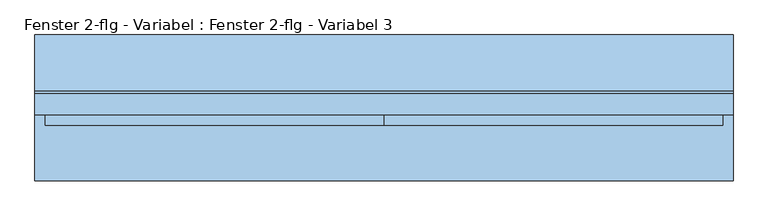
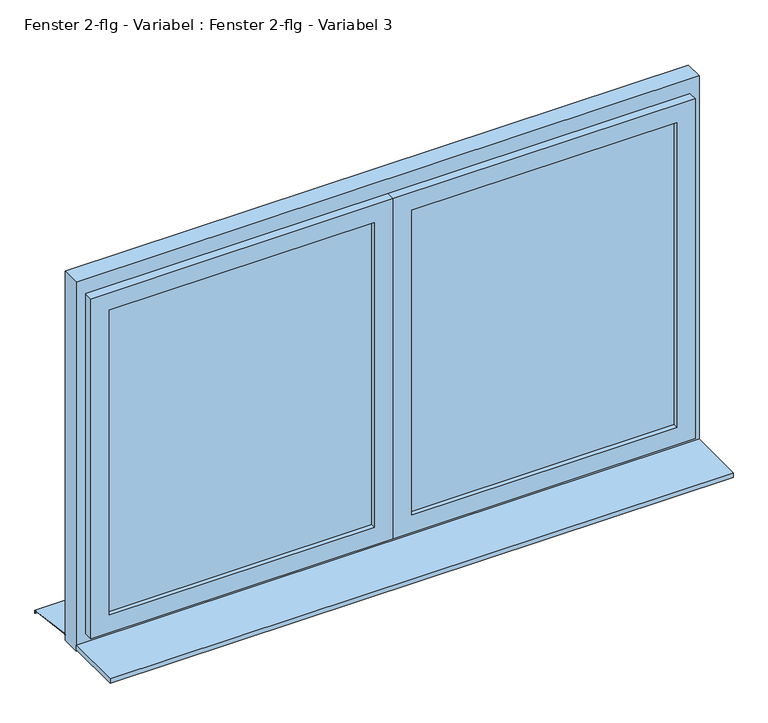
"""IFC4 building model written with IfcOpenShell, lengths in millimetres: window geometry, Fenster 2-flg - Variabel : Fenster 2-flg - Variabel 3."""

from ifc_helpers import new_model, si_unit, frame, origin, place, context, project, spatial, polyline, outline, extrude, faceted_brep, source, transform, mapped, element, save


def fenster_2_flg_variabel_fenster_2_flg_variabel_3_03287464(model_context):
    return source(origin(), model_context, "Body", "SolidModel", [
        extrude(outline(polyline([(60.0, -5.0), (915.0, -5.0), (915.0, -35.0), (60.0, -35.0), (60.0, -5.0)])), frame((0.0, 0.0, 1110.0), z_axis=(0.0, 0.0, 1.0), x_axis=(1.0, 0.0, 0.0)), (0.0, 0.0, 1.0), 1040.0),
        extrude(outline(polyline([(-915.0, -5.0), (-60.0, -5.0), (-60.0, -35.0), (-915.0, -35.0), (-915.0, -5.0)])), frame((0.0, 0.0, 1110.0), z_axis=(0.0, 0.0, 1.0), x_axis=(1.0, 0.0, 0.0)), (0.0, 0.0, 1.0), 1040.0),
        extrude(outline(polyline([(-1005.0, -210.0), (-1005.0, -20.0), (1005.0, -20.0), (1005.0, -210.0), (-1005.0, -210.0)])), frame((0.0, 0.0, 1005.0), z_axis=(0.0, 0.0, 1.0), x_axis=(1.0, 0.0, 0.0)), (0.0, 0.0, 1.0), 15.0),
        extrude(outline(polyline([(50.0221543, 1020.0), (210.0, 1000.0), (210.0, 990.0), (208.0, 990.0), (208.0, 998.3604634), (49.8240723, 1018.0), (40.0, 1018.0), (40.0, 1020.0), (50.0221543, 1020.0)])), frame((-1005.0, 0.0, 0.0), z_axis=(1.0, 0.0, 0.0), x_axis=(0.0, 1.0, 0.0)), (0.0, 0.0, 1.0), 2010.0),
        extrude(outline(polyline([(30.0, -20.0), (-30.0, -20.0), (-30.0, 40.0), (30.0, 40.0), (30.0, -20.0)])), frame((0.0, 0.0, 1080.0), z_axis=(0.0, 0.0, 1.0), x_axis=(1.0, 0.0, 0.0)), (0.0, 0.0, 1.0), 1100.0),
        extrude(outline(polyline([(2260.0, -1005.0), (1000.0, -1005.0), (1000.0, 1005.0), (2260.0, 1005.0), (2260.0, -1005.0)]), holes=[polyline([(2180.0, -945.0), (2180.0, 945.0), (1080.0, 945.0), (1080.0, -945.0), (2180.0, -945.0)])]), frame((0.0, -20.0, 0.0), z_axis=(0.0, 1.0, 0.0), x_axis=(0.0, 0.0, 1.0)), (0.0, 0.0, 1.0), 60.0),
        faceted_brep([(-945.0, -20.0, 1080.0), (-945.0, 10.0, 1080.0), (-30.0, 10.0, 1080.0), (-30.0, -20.0, 1080.0), (-30.0, 10.0, 2180.0), (-30.0, -20.0, 2180.0), (-945.0, 10.0, 2180.0), (-60.0, 10.0, 2150.0), (-915.0, 10.0, 2150.0), (-915.0, 10.0, 1110.0), (-60.0, 10.0, 1110.0), (0.0, -20.0, 1050.0), (-975.0, -20.0, 1050.0), (-975.0, -20.0, 2210.0), (0.0, -20.0, 2210.0), (-945.0, -20.0, 2180.0), (-975.0, -50.0, 1050.0), (0.0, -50.0, 1050.0), (0.0, -50.0, 2210.0), (-975.0, -50.0, 2210.0), (-60.0, -50.0, 1110.0), (-915.0, -50.0, 1110.0), (-915.0, -50.0, 2150.0), (-60.0, -50.0, 2150.0)], [[[0, 1, 2, 3]], [[3, 2, 4, 5]], [[2, 1, 6, 4], [7, 8, 9, 10]], [[11, 12, 13, 14], [5, 15, 0, 3]], [[16, 12, 11, 17]], [[17, 11, 14, 18]], [[18, 19, 16, 17], [20, 21, 22, 23]], [[9, 21, 20, 10]], [[10, 20, 23, 7]], [[15, 6, 1, 0]], [[19, 13, 12, 16]], [[8, 22, 21, 9]], [[5, 4, 6, 15]], [[18, 14, 13, 19]], [[7, 23, 22, 8]]]),
        faceted_brep([(30.0, -20.0, 1080.0), (30.0, 10.0, 1080.0), (945.0, 10.0, 1080.0), (945.0, -20.0, 1080.0), (945.0, 10.0, 2180.0), (945.0, -20.0, 2180.0), (30.0, 10.0, 2180.0), (915.0, 10.0, 2150.0), (60.0, 10.0, 2150.0), (60.0, 10.0, 1110.0), (915.0, 10.0, 1110.0), (975.0, -20.0, 1050.0), (0.0, -20.0, 1050.0), (0.0, -20.0, 2210.0), (975.0, -20.0, 2210.0), (30.0, -20.0, 2180.0), (0.0, -50.0, 1050.0), (975.0, -50.0, 1050.0), (975.0, -50.0, 2210.0), (0.0, -50.0, 2210.0), (915.0, -50.0, 1110.0), (60.0, -50.0, 1110.0), (60.0, -50.0, 2150.0), (915.0, -50.0, 2150.0)], [[[0, 1, 2, 3]], [[3, 2, 4, 5]], [[2, 1, 6, 4], [7, 8, 9, 10]], [[11, 12, 13, 14], [5, 15, 0, 3]], [[16, 12, 11, 17]], [[17, 11, 14, 18]], [[18, 19, 16, 17], [20, 21, 22, 23]], [[9, 21, 20, 10]], [[10, 20, 23, 7]], [[15, 6, 1, 0]], [[19, 13, 12, 16]], [[8, 22, 21, 9]], [[5, 4, 6, 15]], [[18, 14, 13, 19]], [[7, 23, 22, 8]]]),
    ])


if __name__ == "__main__":
    model = new_model("IFC4")
    model_context = context("Model", 3, world=origin())
    ifc_project = project(units=[si_unit("LENGTHUNIT", "METRE", prefix="MILLI")], contexts=[model_context])
    site = spatial("IfcSite", under=ifc_project)
    building = spatial("IfcBuilding", under=site)
    placement = place(None, origin())
    fenster_2_flg_variabel_fenster_2_flg_variabel_3_shape = fenster_2_flg_variabel_fenster_2_flg_variabel_3_03287464(model_context)
    element("IfcWindow", 1, ObjectType="Fenster 2-flg - Variabel : Fenster 2-flg - Variabel 3", at=placement, inside=building, context=model_context, shape_type="MappedRepresentation", body=[
        mapped(fenster_2_flg_variabel_fenster_2_flg_variabel_3_shape, transform((0.0, 0.0, 0.0), x_axis=(1.0, 0.0, 0.0), y_axis=(0.0, 1.0, 0.0), z_axis=(0.0, 0.0, 1.0))),
    ])
    save(model, "model.ifc")

# Revit data of these elements
# Type "Fenster 2-flg - Variabel : Fenster 2-flg - Variabel 3"
#   Type Mark = "53"
#   Operation = "DoublePanelVertical"
#   Construction Type Id = "GSP4R"
#   Keynote = "16.05.01"
#   Analytic Construction = "1/8 Zoll Pilkington-Verglasung einfach"
#   Cost = 130.98
#   Visual Light Transmittance = 0.9
#   Solar Heat Gain Coefficient = 0.78
#   Rough Width [instance default] = 2.010 m
#   Rough Height [instance default] = 1.260 m
#   Heat Transfer Coefficient (U) = 3.6886 W/(m²·K)
#   Rahmentiefe = 0.060 m
#   Rahmenhöhe unten = 0.080 m
#   Höhe oberer  Rahmen = 0.080 m
#   Rahmenbreite = 0.060 m
#   Height [instance default] = 1.260 m
#   Tiefe Flügel = 0.060 m
#   Flügelbreite = 0.060 m
#   Einbautiefe (von außen) [instance default] = 0.140 m
#   Width [instance default] = 2.010 m
#   Define Thermal Properties by = 1
#   Öffnungsrichtung oben [instance default] = yes
#   Öffnungsrichtung in Draufsicht anzeigen [instance default] = no
#   Drehflügel 1 [instance default] = yes
#   Bild [instance default] = none
#   Glas [instance default] = none
#   Fensterflügel [instance default] = none
#   Äußere Fensterbank [instance default] = none
#   Innere Fensterbank [instance default] = none
#   Wall Closure = (empty or 0)
# Element 1 (IfcWindow, "Fenster 2-flg - Variabel : Fenster 2-flg - Variabel 3")
#   Materials on its faces: "Kunststoff - Weiß", "Glas", "Holz - Birke"
# Materials
#   "Kunststoff - Weiß": class "Kunststoff", colour RGB 249 249 249, transparency 0, Cost = 0
#   "Glas": class "Glas", colour RGB 0 0 255, transparency 0.75, Comments = "Render-Darstellung nicht aktualisiert ", Cost = 0
#   "Holz - Birke": class "Holz", colour RGB 213 164 103, transparency 0, Cost = 0
